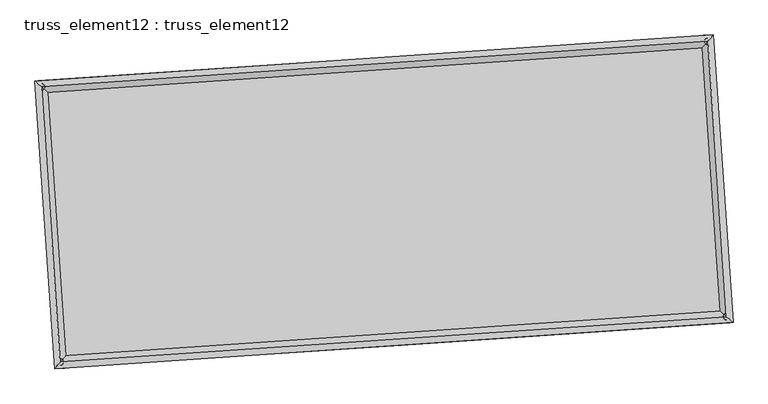
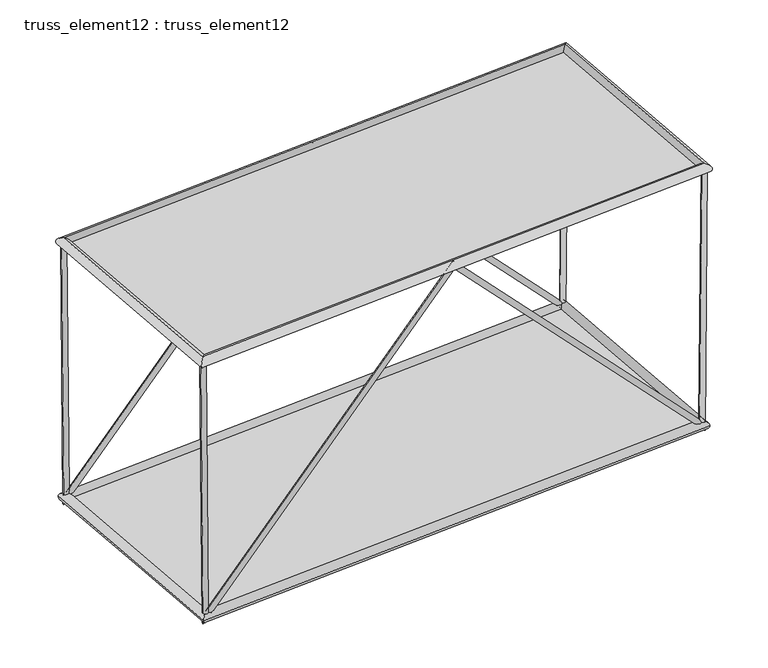
"""IFC4 building model written with IfcOpenShell, lengths in millimetres: plate geometry, truss_element12 : truss_element12."""

import ifcopenshell
import ifcopenshell.guid

model = None  # the IFC model being written
_history = None  # IfcOwnerHistory: only IFC2X3 demands one
_inside = {}  # id of a spatial element -> (the spatial element, [elements in it])
_under = {}  # id of a project, library or spatial element -> (it, [spatial elements below it])
_declared = {}  # id of a project -> (the project, [libraries it declares])
_typed = {}  # id of a type object -> (the type object, [elements of that type])
_made_of = {}  # id of a material, layer set ... -> (it, [elements and type objects made of it])


def new_model(schema):
    """Start an empty IFC model of exactly this schema.

    Asked for "IFC4X3", IfcOpenShell would pick the latest addendum, in which some entities
    have other attributes; the version numbers below select the first issue.
    IFC2X3 requires an IfcOwnerHistory on every rooted entity: one is made here for all.
    """
    global model, _history
    if schema == "IFC4X3":
        model = ifcopenshell.file(schema_version=(4, 3, 0, 0))
    else:
        model = ifcopenshell.file(schema=schema)
    _inside.clear()
    _under.clear()
    _declared.clear()
    _typed.clear()
    _made_of.clear()
    _history = None
    if model.schema == "IFC2X3":
        org = make("IfcOrganization", Name="unknown")
        user = make(
            "IfcPersonAndOrganization",
            ThePerson=make("IfcPerson", FamilyName="unknown"),
            TheOrganization=org,
        )
        app = make(
            "IfcApplication",
            ApplicationDeveloper=org,
            Version="unknown",
            ApplicationFullName="unknown",
            ApplicationIdentifier="unknown",
        )
        _history = make(
            "IfcOwnerHistory",
            OwningUser=user,
            OwningApplication=app,
            ChangeAction="ADDED",
            CreationDate=0,
        )
    return model


def make(cls, **values):
    """One entity of the class cls with the attributes given. An attribute that is None is left unset."""
    return model.create_entity(
        cls, **{name: value for name, value in values.items() if value is not None}
    )


def rooted(cls, **values):
    """An entity with a GlobalId (a new one), such as an element, a storey or a relation."""
    return make(cls, GlobalId=ifcopenshell.guid.new(), OwnerHistory=_history, **values)


def si_unit(unit_type, name, prefix=None):
    """IfcSIUnit, for example si_unit("LENGTHUNIT", "METRE", prefix="MILLI")."""
    return make("IfcSIUnit", UnitType=unit_type, Prefix=prefix, Name=name)


def assignment(units):
    """IfcUnitAssignment: the units of a project."""
    return None if units is None else make("IfcUnitAssignment", Units=units)


def point(xyz):
    """IfcCartesianPoint."""
    return None if xyz is None else make("IfcCartesianPoint", Coordinates=xyz)


def direction(xyz):
    """IfcDirection."""
    return None if xyz is None else make("IfcDirection", DirectionRatios=xyz)


def frame(location, z_axis=None, x_axis=None):
    """IfcAxis2Placement3D, a coordinate frame: its origin and axes. An axis left out is left unset."""
    return make(
        "IfcAxis2Placement3D",
        Location=point(location),
        Axis=direction(z_axis),
        RefDirection=direction(x_axis),
    )


def origin():
    """The frame at (0, 0, 0) with its axes left unset."""
    return frame((0.0, 0.0, 0.0))


def origin_with_axes():
    """The frame at (0, 0, 0) with the z axis (0, 0, 1) and the x axis (1, 0, 0) written out."""
    return frame((0.0, 0.0, 0.0), z_axis=(0.0, 0.0, 1.0), x_axis=(1.0, 0.0, 0.0))


def place(relative_to, where):
    """IfcLocalPlacement: puts the frame where relative to a parent placement (None: the world)."""
    return make(
        "IfcLocalPlacement", PlacementRelTo=relative_to, RelativePlacement=where
    )


def context(
    kind, dimensions, precision=None, world=None, true_north=None, identifier=None
):
    """IfcGeometricRepresentationContext, for example the 3D "Model" context."""
    return make(
        "IfcGeometricRepresentationContext",
        ContextIdentifier=identifier,
        ContextType=kind,
        CoordinateSpaceDimension=dimensions,
        Precision=precision,
        WorldCoordinateSystem=world,
        TrueNorth=true_north,
    )


def project(units=None, contexts=None):
    """IfcProject with its units and contexts."""
    return rooted(
        "IfcProject",
        Name="project",
        RepresentationContexts=contexts,
        UnitsInContext=assignment(units),
    )


def spatial(cls, under=None, at=None, **own):
    """A site, building, storey or space (cls), placed at a placement, below another one or the project."""
    s = rooted(cls, ObjectPlacement=at, **own)
    if under is not None:
        _under.setdefault(under.id(), (under, []))[1].append(s)
    return s


def polyline(points):
    """IfcPolyline through the points."""
    return make("IfcPolyline", Points=[point(p) for p in points])


def circle_curve(where, radius):
    """IfcCircle in the frame where."""
    return make("IfcCircle", Position=where, Radius=radius)


def ellipse_curve(where, semi_axis1, semi_axis2):
    """IfcEllipse in the frame where."""
    return make(
        "IfcEllipse", Position=where, SemiAxis1=semi_axis1, SemiAxis2=semi_axis2
    )


def outline(outer, holes=None, kind="AREA"):
    """IfcArbitraryClosedProfileDef: a profile drawn as a closed curve; with holes, ...WithVoids."""
    if holes is None:
        return make("IfcArbitraryClosedProfileDef", ProfileType=kind, OuterCurve=outer)
    return make(
        "IfcArbitraryProfileDefWithVoids",
        ProfileType=kind,
        OuterCurve=outer,
        InnerCurves=holes,
    )


def extrude(swept, where, along, depth):
    """IfcExtrudedAreaSolid: the profile swept, set in the frame where, extruded along a direction by depth."""
    return make(
        "IfcExtrudedAreaSolid",
        SweptArea=swept,
        Position=where,
        ExtrudedDirection=direction(along),
        Depth=depth,
    )


def shape(context_of_items, identifier, shape_type, items):
    """IfcShapeRepresentation: the items that make up one representation, for example the "Body"."""
    return make(
        "IfcShapeRepresentation",
        ContextOfItems=context_of_items,
        RepresentationIdentifier=identifier,
        RepresentationType=shape_type,
        Items=items,
    )


def source(mapping_origin, context_of_items, identifier, shape_type, items):
    """IfcRepresentationMap: a shape defined once, which mapped items show again and again."""
    return make(
        "IfcRepresentationMap",
        MappingOrigin=mapping_origin,
        MappedRepresentation=shape(context_of_items, identifier, shape_type, items),
    )


def transform(
    local_origin,
    x_axis=None,
    y_axis=None,
    z_axis=None,
    scale=None,
    scale2=None,
    scale3=None,
    uniform=True,
):
    """IfcCartesianTransformationOperator3D, or its non-uniform kind. x_axis, y_axis, z_axis: its Axis1, 2, 3."""
    if uniform:
        return make(
            "IfcCartesianTransformationOperator3D",
            Axis1=direction(x_axis),
            Axis2=direction(y_axis),
            LocalOrigin=point(local_origin),
            Scale=scale,
            Axis3=direction(z_axis),
        )
    return make(
        "IfcCartesianTransformationOperator3DnonUniform",
        Axis1=direction(x_axis),
        Axis2=direction(y_axis),
        LocalOrigin=point(local_origin),
        Scale=scale,
        Axis3=direction(z_axis),
        Scale2=scale2,
        Scale3=scale3,
    )


def mapped(mapping_source, mapping_target):
    """IfcMappedItem: shows the shape of a source again, moved by a transform."""
    return make(
        "IfcMappedItem", MappingSource=mapping_source, MappingTarget=mapping_target
    )


def made_of(thing, what):
    """Note that an element or type object is made of a material, layer set ...; save() writes the relation."""
    if what is not None:
        _made_of.setdefault(what.id(), (what, []))[1].append(thing)
    return thing


def element(
    cls,
    number,
    at=None,
    inside=None,
    cuts=None,
    type_object=None,
    material=None,
    context=None,
    identifier="Body",
    shape_type=None,
    held_by="IfcProductDefinitionShape",
    body=None,
    shapes=None,
    **own,
):
    """One element of the class cls, such as IfcWall. Its Tag is "e" and its number.

    at: its placement. inside: the storey or other place that contains it. cuts: it is an
    opening in that element (IfcRelVoidsElement). A single representation is given by context,
    identifier, shape_type and body (its items); several are given by shapes. held_by: the class
    of the entity that holds the representations. save() writes the other relations.
    """
    e = rooted(cls, Tag="e%d" % number, ObjectPlacement=at, **own)
    if body is not None:
        shapes = [shape(context, identifier, shape_type, body)]
    if shapes is not None:
        e.Representation = make(held_by, Representations=shapes)
    if inside is not None:
        _inside.setdefault(inside.id(), (inside, []))[1].append(e)
    if cuts is not None:
        rooted(
            "IfcRelVoidsElement", RelatingBuildingElement=cuts, RelatedOpeningElement=e
        )
    if type_object is not None:
        _typed.setdefault(type_object.id(), (type_object, []))[1].append(e)
    return made_of(e, material)


def aggregate(whole, parts):
    """IfcRelAggregates: a whole, such as a stair, and the parts it consists of."""
    return rooted("IfcRelAggregates", RelatingObject=whole, RelatedObjects=parts)


def save(model, path):
    """Write the relations noted so far, then the file.

    IfcRelAggregates (storeys below a building ...), IfcRelContainedInSpatialStructure (elements
    in a storey), IfcRelDefinesByType, IfcRelAssociatesMaterial and IfcRelDeclares: one each for
    every whole, place, type object, material and project.
    """
    for whole, parts in _under.values():
        aggregate(whole, parts)
    for where, things in _inside.values():
        rooted(
            "IfcRelContainedInSpatialStructure",
            RelatedElements=things,
            RelatingStructure=where,
        )
    for kind, things in _typed.values():
        rooted("IfcRelDefinesByType", RelatedObjects=things, RelatingType=kind)
    for what, things in _made_of.values():
        rooted("IfcRelAssociatesMaterial", RelatedObjects=things, RelatingMaterial=what)
    for by, libraries in _declared.values():
        rooted("IfcRelDeclares", RelatingContext=by, RelatedDefinitions=libraries)
    model.write(path)


def plane_surface(at):
    """IfcPlane: the flat surface through the origin of the frame at, square to its z axis."""
    return make("IfcPlane", Position=at)


def cylinder_surface(at, radius):
    """IfcCylindricalSurface: all points at the distance radius from the z axis of the frame at."""
    return make("IfcCylindricalSurface", Position=at, Radius=radius)


def advanced_brep(points, edges, surfaces, faces):
    """IfcAdvancedBrep: a solid bounded by faces that lie on surfaces and meet in shared edges.

    An edge is (start, end): straight between two places in points (the first is 0);
    or (start, end, curve); or (start, end, curve, False) where it runs against its curve.
    A face is (place in surfaces, loops), or (place, loops, False) where it looks against
    its surface's normal. A loop lists edges by number (the first is 1), with a minus sign
    where the edge is run from its end to its start. The first loop is the outer one.
    """
    corners = [point(p) for p in points]
    vertices = [make("IfcVertexPoint", VertexGeometry=c) for c in corners]
    made = []
    for start, end, *more in edges:
        made.append(
            make(
                "IfcEdgeCurve",
                EdgeStart=vertices[start],
                EdgeEnd=vertices[end],
                EdgeGeometry=more[0] if more else make("IfcPolyline", Points=[corners[start], corners[end]]),
                SameSense=more[1] if len(more) > 1 else True,
            )
        )
    hull = []
    for where, loops, *sense in faces:
        bounds = []
        for j, loop in enumerate(loops):
            ring = [make("IfcOrientedEdge", EdgeElement=made[abs(k) - 1], Orientation=k > 0) for k in loop]
            bounds.append(
                make(
                    "IfcFaceOuterBound" if j == 0 else "IfcFaceBound",
                    Bound=make("IfcEdgeLoop", EdgeList=ring),
                    Orientation=True,
                )
            )
        hull.append(make("IfcAdvancedFace", Bounds=bounds, FaceSurface=surfaces[where], SameSense=sense[0] if sense else True))
    return make("IfcAdvancedBrep", Outer=make("IfcClosedShell", CfsFaces=hull))


def truss_element12_truss_element12_f6fe5973(model_context):
    return source(origin(), model_context, "Body", "SolidModel", [
        advanced_brep(
        [(-3710.2419701, 2273.1351163, 5000.2468963), (-3809.3412307, 2259.7741453, 4999.3408025), (-3666.054382, 2276.1481, 123.0325372), (-3762.9325009, 2262.9385801, -123.0325372), (1064.1133725, 2598.6802581, 5071.9126382), (1064.5556921, 2592.106649, 4927.6678811), (5793.5123498, 2921.1599962, 123.0270149), (5891.2486273, 2921.2204923, -123.0270149), (5838.4629041, 2924.2250036, 5000.2475381), (5938.4584258, 2924.439549, 4999.3258017)],
        [
            (0, 1, circle_curve(frame((-3759.7916004, 2266.4546308, 4999.7938494), z_axis=(-0.009059631795656001, -0.0006177418532641554, 0.9999587698834037), x_axis=(-0.13360979880213997, 0.991033835814136, -0.0005982771700932393)), 50.0)),
            (1, 0, circle_curve(frame((-3759.7916004, 2266.4546308, 4999.7938494), z_axis=(-0.009059631795656001, -0.0006177418532641554, 0.9999587698834037), x_axis=(-0.13360979880213997, 0.991033835814136, -0.0005982771700932393)), 50.0)),
            (0, 2),
            (2, 3, ellipse_curve(frame((-3714.4934414, 2269.54334, 0.0), z_axis=(-0.9274570070583217, -0.06323976771716287, 0.3685433920686947), x_axis=(0.36768962300005015, 0.02507135767326109, 0.9296105464991781)), 132.6366613, 50.0)),
            (3, 1),
            (3, 2, ellipse_curve(frame((-3714.4934414, 2269.54334, 0.0), z_axis=(-0.9274570070583217, -0.06323976771716287, 0.3685433920686947), x_axis=(0.36768962300005015, 0.02507135767326109, 0.9296105464991781)), 132.6366613, 50.0)),
            (2, 4),
            (4, 5, ellipse_curve(frame((1064.3345323, 2595.3934535, 4999.7902597), z_axis=(-0.9976833952413823, -0.06802823817187122, 4.0876142565046614e-05), x_axis=(-4.078144873295169e-05, -2.7807319613378337e-06, -0.9999999991645705)), 72.2794243, 50.0)),
            (5, 3),
            (5, 4, ellipse_curve(frame((1064.3345323, 2595.3934535, 4999.7902597), z_axis=(-0.9976833952413823, -0.06802823817187122, 4.0876142565046614e-05), x_axis=(-4.078144873295169e-05, -2.7807319613378337e-06, -0.9999999991645705)), 72.2794243, 50.0)),
            (4, 6),
            (6, 7, ellipse_curve(frame((5842.3804885, 2921.1902443, 0.0), z_axis=(-0.9275008521416513, -0.06324275734672206, -0.3684325215282904), x_axis=(-0.36757900930277465, -0.025063815345731454, 0.9296544933900474)), 132.6244381, 50.0)),
            (7, 5),
            (7, 6, ellipse_curve(frame((5842.3804885, 2921.1902443, 0.0), z_axis=(-0.9275008521416513, -0.06324275734672206, -0.3684325215282904), x_axis=(-0.36757900930277465, -0.025063815345731454, 0.9296544933900474)), 132.6244381, 50.0)),
            (8, 9, circle_curve(frame((5888.4606649, 2924.3322763, 4999.7866699), z_axis=(0.009216035288573994, 0.0006284064128948841, 0.9999573339892758), x_axis=(-0.0021511542640449003, 0.9999975010640975, -0.0006086056957160734)), 50.0)),
            (9, 8, circle_curve(frame((5888.4606649, 2924.3322763, 4999.7866699), z_axis=(0.009216035288573994, 0.0006284064128948841, 0.9999573339892758), x_axis=(-0.0021511542640449003, 0.9999975010640975, -0.0006086056957160734)), 50.0)),
            (6, 8),
            (9, 7),
        ],
        [
            plane_surface(frame((-3759.7916004, 2316.4546212, 4999.8247378), z_axis=(-0.00905963179565723, -0.0006177418532678904, 0.9999587698834038), x_axis=(0.9999589606937513, -5.596743421598659e-06, 0.00905963006691479))),
            cylinder_surface(frame((-3759.7916004, 2266.4546308, 4999.7938494), z_axis=(-0.009059631795656003, -0.0006177418532641555, 0.9999587698834039), x_axis=(-0.13360979880213997, 0.991033835814136, -0.0005982771700932393)), 50.0),
            cylinder_surface(frame((-3714.4934414, 2269.54334, 0.0), z_axis=(-0.6901867139153417, -0.04706120837656332, -0.7220993993910259), x_axis=(-0.020415334139245483, 0.9987521360670553, -0.0455783373268222)), 50.0),
            cylinder_surface(frame((1064.3345323, 2595.3934535, 4999.7902597), z_axis=(-0.6901278150897087, -0.047057192289543075, 0.7221559523353178), x_axis=(-0.11534924188526842, 0.9922789537754221, -0.04557444778434232)), 50.0),
            plane_surface(frame((5888.4606649, 2874.3322862, 4999.8180916), z_axis=(0.009216035288575347, 0.0006284064128996202, 0.9999573339892759), x_axis=(0.9999575314449909, -5.7916616409414675e-06, -0.009216033468739223))),
            cylinder_surface(frame((5842.3804885, 2921.1902443, 0.0), z_axis=(-0.009216035288573994, -0.0006284064128948841, -0.9999573339892758), x_axis=(-0.0021511542640449003, 0.9999975010640975, -0.0006086056957160734)), 50.0),
        ],
        [
            (0, [[1, 2]]),
            (1, [[-1, 3, 4, 5]]),
            (1, [[-2, -5, 6, -3]]),
            (2, [[-4, 7, 8, 9]]),
            (2, [[-6, -9, 10, -7]]),
            (3, [[-8, 11, 12, 13]]),
            (3, [[-10, -13, 14, -11]]),
            (4, [[15, 16]]),
            (5, [[-12, 17, -16, 18]]),
            (5, [[-14, -18, -15, -17]]),
        ],
    ),
        advanced_brep(
        [(-3438.1290172, -1717.598468, 5000.2468963), (-3537.2282778, -1730.959439, 4999.3408025), (-3393.941429, -1714.5854843, 123.0325372), (-3490.819548, -1727.7950042, -123.0325372), (1336.2263254, -1392.0533262, 5071.9126382), (1336.668645, -1398.6269353, 4927.6678811), (6065.6253027, -1069.5735881, 123.0270149), (6163.3615802, -1069.513092, -123.0270149), (6110.575857, -1066.5085807, 5000.2475381), (6210.5713787, -1066.2940353, 4999.3258017)],
        [
            (0, 1, circle_curve(frame((-3487.6786475, -1724.2789535, 4999.7938494), z_axis=(-0.009059631795655944, -0.0006177418532642077, 0.9999587698834038), x_axis=(-0.13360979880213966, 0.991033835814136, -0.0005982771700931769)), 50.0)),
            (1, 0, circle_curve(frame((-3487.6786475, -1724.2789535, 4999.7938494), z_axis=(-0.009059631795655944, -0.0006177418532642077, 0.9999587698834038), x_axis=(-0.13360979880213966, 0.991033835814136, -0.0005982771700931769)), 50.0)),
            (0, 2),
            (2, 3, ellipse_curve(frame((-3442.3804885, -1721.1902443, 0.0), z_axis=(-0.9274570070583221, -0.06323976771716276, 0.3685433920686939), x_axis=(0.3676896230000495, 0.025071357673260925, 0.9296105464991783)), 132.6366613, 50.0)),
            (3, 1),
            (3, 2, ellipse_curve(frame((-3442.3804885, -1721.1902443, 0.0), z_axis=(-0.9274570070583221, -0.06323976771716276, 0.3685433920686939), x_axis=(0.3676896230000495, 0.025071357673260925, 0.9296105464991783)), 132.6366613, 50.0)),
            (2, 4),
            (4, 5, ellipse_curve(frame((1336.4474852, -1395.3401308, 4999.7902597), z_axis=(-0.9976833952413823, -0.06802823817187109, 4.0876142564083687e-05), x_axis=(-4.07814487320292e-05, -2.7807319611648704e-06, -0.9999999991645705)), 72.2794243, 50.0)),
            (5, 3),
            (5, 4, ellipse_curve(frame((1336.4474852, -1395.3401308, 4999.7902597), z_axis=(-0.9976833952413823, -0.06802823817187109, 4.0876142564083687e-05), x_axis=(-4.07814487320292e-05, -2.7807319611648704e-06, -0.9999999991645705)), 72.2794243, 50.0)),
            (4, 6),
            (6, 7, ellipse_curve(frame((6114.4934414, -1069.54334, 0.0), z_axis=(-0.9275008521416513, -0.06324275734672197, -0.3684325215282904), x_axis=(-0.36757900930277465, -0.02506381534573148, 0.9296544933900474)), 132.6244381, 50.0)),
            (7, 5),
            (7, 6, ellipse_curve(frame((6114.4934414, -1069.54334, 0.0), z_axis=(-0.9275008521416513, -0.06324275734672197, -0.3684325215282904), x_axis=(-0.36757900930277465, -0.02506381534573148, 0.9296544933900474)), 132.6244381, 50.0)),
            (8, 9, circle_curve(frame((6160.5736179, -1066.401308, 4999.7866699), z_axis=(0.009216035288574044, 0.0006284064128948374, 0.9999573339892759), x_axis=(-0.0021511542640451015, 0.9999975010640975, -0.0006086056957160248)), 50.0)),
            (9, 8, circle_curve(frame((6160.5736179, -1066.401308, 4999.7866699), z_axis=(0.009216035288574044, 0.0006284064128948374, 0.9999573339892759), x_axis=(-0.0021511542640451015, 0.9999975010640975, -0.0006086056957160248)), 50.0)),
            (6, 8),
            (9, 7),
        ],
        [
            plane_surface(frame((-3487.6786475, -1674.2789631, 4999.8247378), z_axis=(-0.00905963179565723, -0.0006177418532678904, 0.9999587698834038), x_axis=(0.9999589606937513, -5.596743421598659e-06, 0.00905963006691479))),
            cylinder_surface(frame((-3487.6786475, -1724.2789535, 4999.7938494), z_axis=(-0.009059631795655944, -0.0006177418532642077, 0.9999587698834038), x_axis=(-0.13360979880213966, 0.991033835814136, -0.0005982771700931769)), 50.0),
            cylinder_surface(frame((-3442.3804885, -1721.1902443, 0.0), z_axis=(-0.6901867139153405, -0.04706120837656307, -0.7220993993910272), x_axis=(-0.02041533413924536, 0.9987521360670553, -0.04557833732682192)), 50.0),
            cylinder_surface(frame((1336.4474852, -1395.3401308, 4999.7902597), z_axis=(-0.6901278150897087, -0.047057192289543054, 0.7221559523353177), x_axis=(-0.11534924188526818, 0.992278953775422, -0.04557444778434213)), 50.0),
            plane_surface(frame((6160.5736179, -1116.4012981, 4999.8180916), z_axis=(0.009216035288575347, 0.000628406412899621, 0.9999573339892759), x_axis=(0.9999575314449909, -5.791661640497378e-06, -0.009216033468739223))),
            cylinder_surface(frame((6114.4934414, -1069.54334, 0.0), z_axis=(-0.009216035288574044, -0.0006284064128948374, -0.9999573339892759), x_axis=(-0.0021511542640451015, 0.9999975010640975, -0.0006086056957160248)), 50.0),
        ],
        [
            (0, [[1, 2]]),
            (1, [[-1, 3, 4, 5]]),
            (1, [[-2, -5, 6, -3]]),
            (2, [[-4, 7, 8, 9]]),
            (2, [[-6, -9, 10, -7]]),
            (3, [[-8, 11, 12, 13]]),
            (3, [[-10, -13, 14, -11]]),
            (4, [[15, 16]]),
            (5, [[-12, 17, -16, 18]]),
            (5, [[-14, -18, -15, -17]]),
        ],
    ),
        advanced_brep(
        [(-3487.6805382, -1724.2810491, 4909.7938494), (-3487.6767568, -1724.276858, 5089.7938494), (-3759.7894427, 2266.4528113, 5089.7938494), (-3759.7937581, 2266.4564503, 4909.7938494), (5888.4589075, 2924.3301899, 5089.7866699), (5888.4624223, 2924.3343628, 4909.78667), (6160.5715935, -1066.3994794, 5089.7866699), (6160.5756422, -1066.4031366, 4909.78667)],
        [
            (0, 1, ellipse_curve(frame((-3487.6786475, -1724.2789535, 4999.7938494), z_axis=(-0.7535719234052624, 0.6573654662780954, 5.249543265090631e-07), x_axis=(-0.6573654662778877, -0.7535719234054434, 5.249543265091374e-07)), 127.2792206, 90.0)),
            (1, 2),
            (2, 3, ellipse_curve(frame((-3759.7916004, 2266.4546308, 4999.7938494), z_axis=(-0.6573654662778875, -0.7535719234054435, 5.249543277760535e-07), x_axis=(0.7535719234052622, -0.6573654662780956, -5.249543277759792e-07)), 127.2792206, 90.0)),
            (3, 0),
            (1, 0, ellipse_curve(frame((-3487.6786475, -1724.2789535, 4999.7938494), z_axis=(-0.7535719234052624, 0.6573654662780954, 5.249543265090631e-07), x_axis=(-0.6573654662778877, -0.7535719234054434, 5.249543265091374e-07)), 127.2792206, 90.0)),
            (3, 2, ellipse_curve(frame((-3759.7916004, 2266.4546308, 4999.7938494), z_axis=(-0.6573654662778875, -0.7535719234054435, 5.249543277760535e-07), x_axis=(0.7535719234052622, -0.6573654662780956, -5.249543277759792e-07)), 127.2792206, 90.0)),
            (2, 4),
            (4, 5, ellipse_curve(frame((5888.4606649, 2924.3322763, 4999.7866699), z_axis=(-0.7535719234052609, 0.6573654662780971, 5.2495432471324e-07), x_axis=(-0.6573654662778895, -0.7535719234054419, 5.249543308387929e-07)), 127.2792206, 90.0)),
            (5, 3),
            (5, 4, ellipse_curve(frame((5888.4606649, 2924.3322763, 4999.7866699), z_axis=(-0.7535719234052609, 0.6573654662780971, 5.2495432471324e-07), x_axis=(-0.6573654662778895, -0.7535719234054419, 5.249543308387929e-07)), 127.2792206, 90.0)),
            (4, 6),
            (6, 7, ellipse_curve(frame((6160.5736179, -1066.401308, 4999.7866699), z_axis=(0.6573654662778894, 0.753571923405442, -5.249543295718767e-07), x_axis=(-0.7535719234052608, 0.6573654662780972, 5.249543234463237e-07)), 127.2792206, 90.0)),
            (7, 5),
            (7, 6, ellipse_curve(frame((6160.5736179, -1066.401308, 4999.7866699), z_axis=(0.6573654662778894, 0.753571923405442, -5.249543295718767e-07), x_axis=(-0.7535719234052608, 0.6573654662780972, 5.249543234463237e-07)), 127.2792206, 90.0)),
            (6, 1),
            (0, 7),
        ],
        [
            cylinder_surface(frame((-3487.6786475, -1724.2789535, 4999.7938494), z_axis=(0.06802823822869923, -0.9976833960748769, 0.0), x_axis=(-0.9976833958213659, -0.06802823821141327, 2.254327394957503e-05)), 90.0),
            cylinder_surface(frame((-3759.7916004, 2266.4546308, 4999.7938494), z_axis=(-0.9976833960746017, -0.06802823822868122, 7.423975299672935e-07), x_axis=(-0.06802823819638637, 0.9976833958388891, 2.1800876419784193e-05)), 90.0),
            cylinder_surface(frame((5888.4606649, 2924.3322763, 4999.7866699), z_axis=(-0.0680282382286945, 0.9976833960748772, 0.0), x_axis=(0.9976833958536611, 0.0680282382136106, 2.1058478894324835e-05)), 90.0),
            cylinder_surface(frame((6160.5736179, -1066.401308, 4999.7866699), z_axis=(0.9976833960746018, 0.06802823822868093, -7.423975281756036e-07), x_axis=(0.06802823822868093, -0.9976833958366871, 2.180087642665553e-05)), 90.0),
        ],
        [
            (0, [[1, 2, 3, 4]]),
            (0, [[5, -4, 6, -2]]),
            (1, [[-3, 7, 8, 9]]),
            (1, [[-6, -9, 10, -7]]),
            (2, [[-8, 11, 12, 13]]),
            (2, [[-10, -13, 14, -11]]),
            (3, [[-12, 15, -1, 16]]),
            (3, [[-14, -16, -5, -15]]),
        ],
    ),
        advanced_brep(
        [(-3358.7115243, -1625.2761972, 0.0), (-3526.0494527, -1817.1042913, 0.0), (-3810.4074885, 2353.2123043, 0.0), (-3618.5793943, 2185.8743758, 0.0), (5926.0494527, 3017.1042913, 0.0), (5758.7115243, 2825.2761972, 0.0), (6210.4074885, -1153.2123043, 0.0), (6018.5793943, -985.8743758, 0.0)],
        [
            (0, 1, ellipse_curve(frame((-3442.3804885, -1721.1902443, 0.0), z_axis=(-0.7535719234054598, 0.6573654662780787, 0.0), x_axis=(-0.6573654662780787, -0.7535719234054599, 0.0)), 127.2792206, 90.0)),
            (1, 2),
            (2, 3, ellipse_curve(frame((-3714.4934414, 2269.54334, 0.0), z_axis=(-0.6573654662780787, -0.7535719234054599, 0.0), x_axis=(0.7535719234054599, -0.6573654662780785, 0.0)), 127.2792206, 90.0)),
            (3, 0),
            (1, 0, ellipse_curve(frame((-3442.3804885, -1721.1902443, 0.0), z_axis=(-0.7535719234054598, 0.6573654662780787, 0.0), x_axis=(-0.6573654662780787, -0.7535719234054599, 0.0)), 127.2792206, 90.0)),
            (3, 2, ellipse_curve(frame((-3714.4934414, 2269.54334, 0.0), z_axis=(-0.6573654662780787, -0.7535719234054599, 0.0), x_axis=(0.7535719234054599, -0.6573654662780785, 0.0)), 127.2792206, 90.0)),
            (2, 4),
            (4, 5, ellipse_curve(frame((5842.3804885, 2921.1902443, 0.0), z_axis=(-0.7535719234054583, 0.6573654662780803, 0.0), x_axis=(-0.6573654662780803, -0.7535719234054582, 0.0)), 127.2792206, 90.0)),
            (5, 3),
            (5, 4, ellipse_curve(frame((5842.3804885, 2921.1902443, 0.0), z_axis=(-0.7535719234054583, 0.6573654662780803, 0.0), x_axis=(-0.6573654662780803, -0.7535719234054582, 0.0)), 127.2792206, 90.0)),
            (4, 6),
            (6, 7, ellipse_curve(frame((6114.4934414, -1069.54334, 0.0), z_axis=(0.6573654662780805, 0.7535719234054583, 0.0), x_axis=(-0.7535719234054584, 0.6573654662780803, 0.0)), 127.2792206, 90.0)),
            (7, 5),
            (7, 6, ellipse_curve(frame((6114.4934414, -1069.54334, 0.0), z_axis=(0.6573654662780805, 0.7535719234054583, 0.0), x_axis=(-0.7535719234054584, 0.6573654662780803, 0.0)), 127.2792206, 90.0)),
            (6, 1),
            (0, 7),
        ],
        [
            cylinder_surface(frame((-3442.3804885, -1721.1902443, 0.0), z_axis=(0.06802823822870352, -0.9976833960748764, 0.0), x_axis=(-0.9976833960748764, -0.06802823822870352, 0.0)), 90.0),
            cylinder_surface(frame((-3714.4934414, 2269.54334, 0.0), z_axis=(-0.9976833960748764, -0.06802823822870463, 0.0), x_axis=(-0.06802823822870463, 0.9976833960748764, 0.0)), 90.0),
            cylinder_surface(frame((5842.3804885, 2921.1902443, 0.0), z_axis=(-0.0680282382286991, 0.9976833960748769, 0.0), x_axis=(0.9976833960748769, 0.0680282382286991, 0.0)), 90.0),
            cylinder_surface(frame((6114.4934414, -1069.54334, 0.0), z_axis=(0.9976833960748764, 0.06802823822870442, 0.0), x_axis=(0.06802823822870442, -0.9976833960748764, 0.0)), 90.0),
        ],
        [
            (0, [[1, 2, 3, 4]]),
            (0, [[5, -4, 6, -2]]),
            (1, [[-3, 7, 8, 9]]),
            (1, [[-6, -9, 10, -7]]),
            (2, [[-8, 11, 12, 13]]),
            (2, [[-10, -13, 14, -11]]),
            (3, [[-12, 15, -1, 16]]),
            (3, [[-14, -16, -5, -15]]),
        ],
    ),
        extrude(outline(polyline([(-3442.3804885, -1721.1902443), (-3714.4934414, 2269.54334), (5842.3804885, 2921.1902443), (6114.4934414, -1069.54334), (-3442.3804885, -1721.1902443)])), origin_with_axes(), (0.0, 0.0, 1.0), 20.0),
        extrude(outline(polyline([(-2000.0, 4835.3276717), (2000.0, 4835.3276717), (2000.0, -4835.3276717), (-2000.0, -4835.3276718), (-2000.0, 4835.3276717)])), frame((1200.3910087, 600.0266614, 4999.7902597), z_axis=(7.406776889353197e-07, 5.050399602901239e-08, 0.9999999999997244), x_axis=(-0.06802823822870309, 0.9976833960748765, 0.0)), (0.0, 0.0, 1.0), 20.0),
    ])


if __name__ == "__main__":
    model = new_model("IFC4")
    model_context = context("Model", 3, world=origin())
    ifc_project = project(units=[si_unit("LENGTHUNIT", "METRE", prefix="MILLI")], contexts=[model_context])
    site = spatial("IfcSite", under=ifc_project)
    building = spatial("IfcBuilding", under=site)
    placement = place(None, origin())
    truss_element12_truss_element12_shape = truss_element12_truss_element12_f6fe5973(model_context)
    element("IfcPlate", 1, ObjectType="truss_element12 : truss_element12", at=placement, inside=building, context=model_context, shape_type="MappedRepresentation", body=[
        mapped(truss_element12_truss_element12_shape, transform((0.0, 0.0, 0.0), x_axis=(1.0, 0.0, 0.0), y_axis=(0.0, 1.0, 0.0), z_axis=(0.0, 0.0, 1.0))),
    ])
    save(model, "model.ifc")

# Revit data of these elements
# Type "truss_element12 : truss_element12"
#   steellbar1 = 90 mm
#   steelbar2 = 50 mm
#   offset1 = 5000 mm
#   M = Default Roof
# Element 1 (IfcPlate, "truss_element12 : truss_element12")
#   Materials on its faces: "Default Roof"
# Materials
#   "Default Roof": class "Miscellaneous", colour RGB 0 127 0, transparency 0, Comments = "Rendering appearance not upgraded Rendering appearance not upgraded ", Cost = 0
